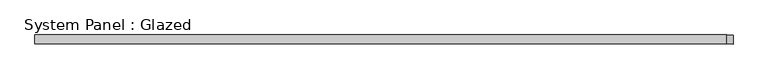
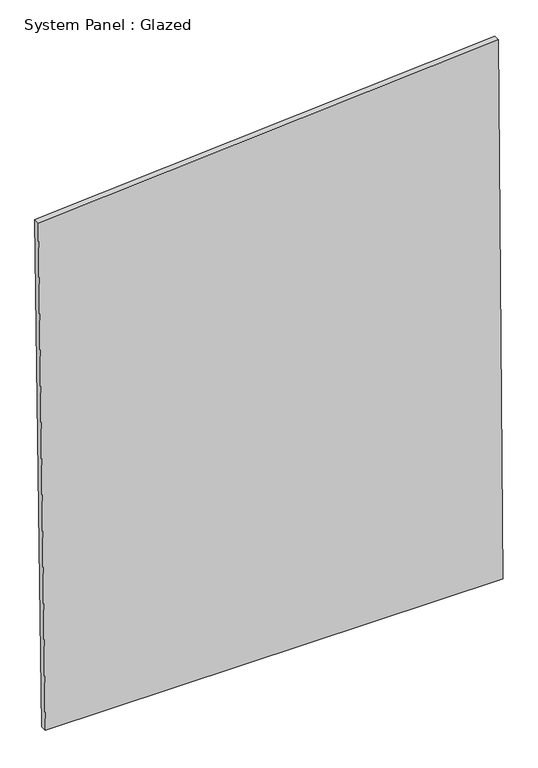
"""IFC4 building model written with IfcOpenShell, lengths in millimetres: plate geometry, System Panel : Glazed."""

from ifc_helpers import new_model, si_unit, frame, origin, place, context, project, spatial, polyline, outline, extrude, source, transform, mapped, element, save


def system_panel_glazed_3b9d15b0(model_context):
    return source(origin(), model_context, "Body", "SweptSolid", [
        extrude(outline(polyline([(0.0, -942.7108166), (0.0, 972.0020553), (2391.8329241, 954.5438482), (2255.5087034, -972.0020553), (0.0, -942.7108166)])), frame((0.0, -49.5, 0.0), z_axis=(0.0, 1.0, 0.0), x_axis=(0.0, 0.0, 1.0)), (0.0, 0.0, 1.0), 25.0),
    ])


if __name__ == "__main__":
    model = new_model("IFC4")
    model_context = context("Model", 3, world=origin())
    ifc_project = project(units=[si_unit("LENGTHUNIT", "METRE", prefix="MILLI")], contexts=[model_context])
    site = spatial("IfcSite", under=ifc_project)
    building = spatial("IfcBuilding", under=site)
    placement = place(None, origin())
    system_panel_glazed_shape = system_panel_glazed_3b9d15b0(model_context)
    element("IfcPlate", 1, ObjectType="System Panel : Glazed", at=placement, inside=building, context=model_context, shape_type="MappedRepresentation", body=[
        mapped(system_panel_glazed_shape, transform((0.0, 0.0, 0.0), x_axis=(1.0, 0.0, 0.0), y_axis=(0.0, 1.0, 0.0), z_axis=(0.0, 0.0, 1.0))),
    ])
    save(model, "model.ifc")

# Revit data of these elements
# Element 1 (IfcPlate, "System Panel : Glazed")
#   Materials on its faces: "Glass, Clear Glazing"
# Materials
#   "Glass, Clear Glazing": class "Glass", colour RGB 247 249 248, transparency 0.85, Description = "Clear glazing", Cost = 0
